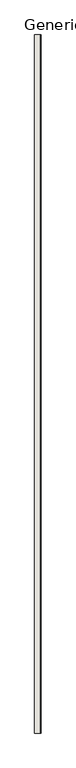
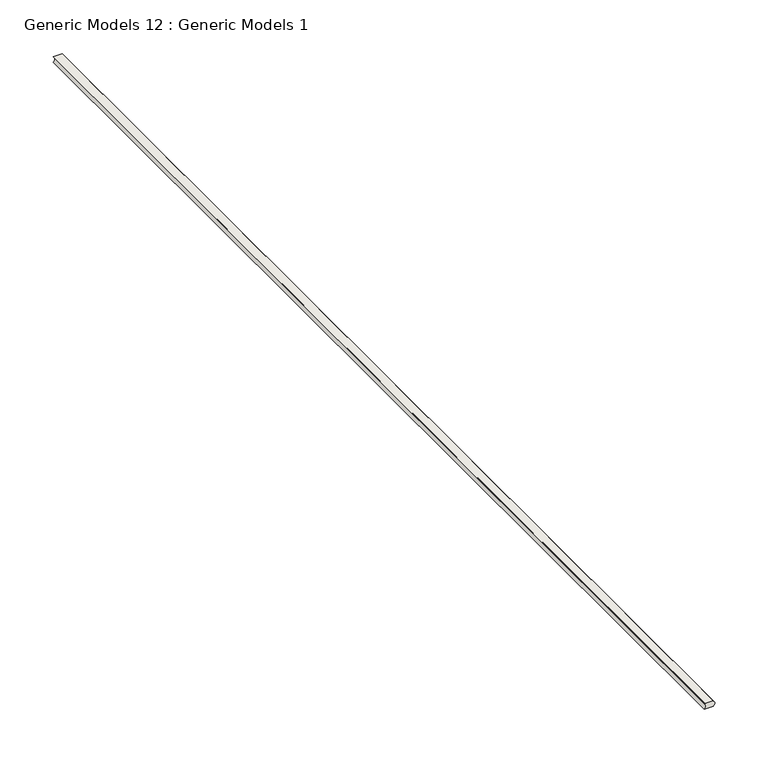
"""IFC4 building model written with IfcOpenShell, lengths in millimetres: wall geometry, Generic Models 12 : Generic Models 1."""

from ifc_helpers import new_model, si_unit, point, frame, frame_2d, origin, place, context, project, spatial, polyline, circle_curve, trimmed, segment, composite_curve, outline, extrude, source, transform, mapped, element, save


def generic_models_12_generic_models_1_17250769(model_context):
    return source(origin(), model_context, "Body", "SweptSolid", [
        extrude(outline(composite_curve([segment(trimmed(circle_curve(frame_2d((2454.275, 136239.5102595)), 4.3100275), [point((2457.45, 136242.425))], [point((2451.1, 136242.425))], True, "CARTESIAN"), True, "CONTINUOUS"), segment(polyline([(2451.1, 136242.425), (2451.1, 136251.95)]), True, "CONTINUOUS"), segment(trimmed(circle_curve(frame_2d((2454.275, 136249.0352595)), 4.3100275), [point((2451.1, 136251.95))], [point((2457.45, 136251.95))], False, "CARTESIAN"), True, "CONTINUOUS"), segment(polyline([(2457.45, 136251.95), (2457.45, 136242.425)]), True, "CONTINUOUS")], self_intersect=False)), frame((0.0, 0.0, 0.0), z_axis=(0.0, 1.0, 0.0), x_axis=(0.0, 0.0, 1.0)), (0.0, 0.0, 1.0), 1219.2),
    ])


if __name__ == "__main__":
    model = new_model("IFC4")
    model_context = context("Model", 3, world=origin())
    ifc_project = project(units=[si_unit("LENGTHUNIT", "METRE", prefix="MILLI")], contexts=[model_context])
    site = spatial("IfcSite", under=ifc_project)
    building = spatial("IfcBuilding", under=site)
    placement = place(None, origin())
    generic_models_12_generic_models_1_shape = generic_models_12_generic_models_1_17250769(model_context)
    element("IfcWall", 1, ObjectType="Generic Models 12 : Generic Models 1", at=placement, inside=building, context=model_context, shape_type="MappedRepresentation", body=[
        mapped(generic_models_12_generic_models_1_shape, transform((0.0, 0.0, 0.0), x_axis=(1.0, 0.0, 0.0), y_axis=(0.0, 1.0, 0.0), z_axis=(0.0, 0.0, 1.0))),
    ])
    save(model, "model.ifc")

# Revit data of these elements
# Element 1 (IfcWall, "Generic Models 12 : Generic Models 1")
#   Materials on its faces: "ACOUSTICAL SEALANT"
# Materials
#   "ACOUSTICAL SEALANT": class "Unassigned", colour RGB 120 120 120, transparency 0, Cost = 0
